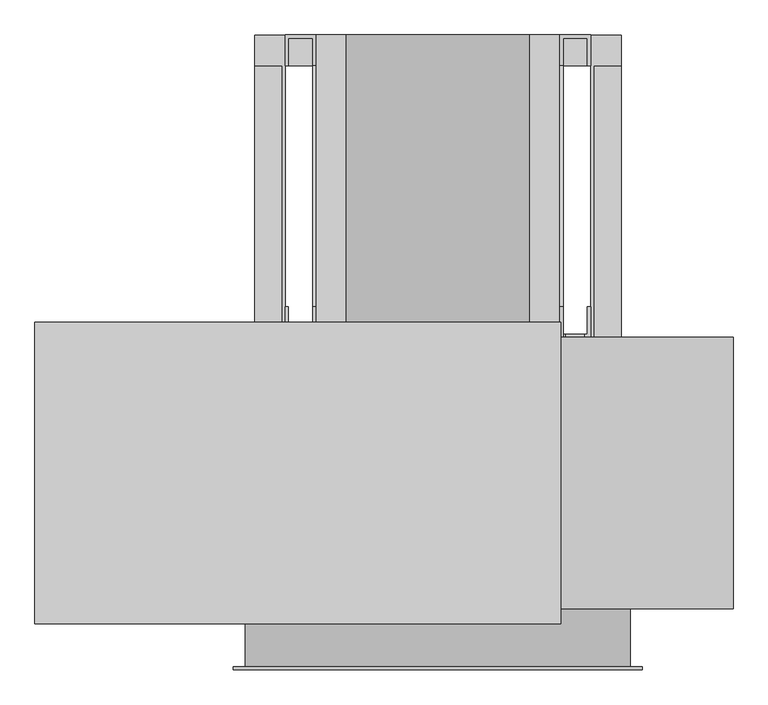
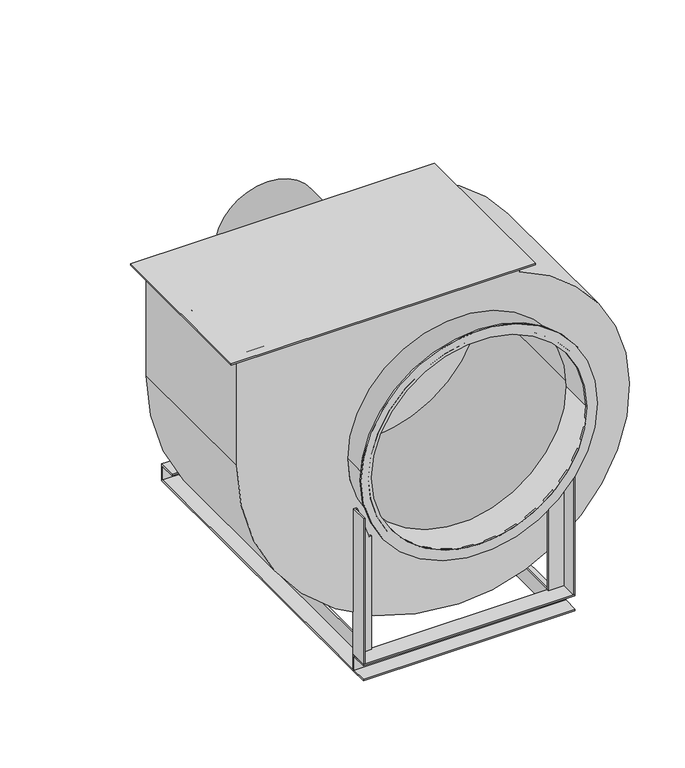
"""IFC4 building model written with IfcOpenShell, lengths in millimetres: proxy geometry, ВЕЗА_Вентилятор ВРАН : ВРАН6-063-ПО."""

from ifc_helpers import new_model, si_unit, point, frame, frame_2d, origin, place, context, project, spatial, polyline, circle_curve, trimmed, segment, composite_curve, outline, extrude, faceted_brep, source, transform, mapped, element, save


def mechanical_equipment_27ed4517(model_context):
    return source(origin(), model_context, "Body", "SolidModel", [
        extrude(outline(polyline([(201.5, 247.0), (201.5, -247.0), (-659.5, -247.0), (-659.5, 247.0), (201.5, 247.0)])), frame((0.0, 0.0, 1055.0), z_axis=(0.0, 0.0, 1.0), x_axis=(1.0, 0.0, 0.0)), (0.0, 0.0, 1.0), 5.0),
        extrude(outline(composite_curve([segment(trimmed(circle_curve(frame_2d((730.0, 5.524027)), 635.024027), [point((730.0, -629.5))], [point((95.0, 0.0))], False, "CARTESIAN"), True, "CONTINUOUS"), segment(trimmed(circle_curve(frame_2d((578.1699763, 0.3189338)), 483.1700816), [point((95.0, 0.0))], [point((1030.0, 171.5))], False, "CARTESIAN"), True, "CONTINUOUS"), segment(polyline([(1030.0, 171.5), (1060.0, 171.5), (1060.0, -629.5), (730.0, -629.5)]), True, "CONTINUOUS")], self_intersect=False), holes=[composite_curve([segment(trimmed(circle_curve(frame_2d((640.0, 0.0)), 315.0), [point((640.0, -315.0))], [point((640.0, 315.0))], True, "CARTESIAN"), True, "CONTINUOUS"), segment(trimmed(circle_curve(frame_2d((640.0, 0.0)), 315.0), [point((640.0, 315.0))], [point((640.0, -315.0))], True, "CARTESIAN"), True, "CONTINUOUS")], self_intersect=False)]), frame((0.0, -222.0, 0.0), z_axis=(0.0, 1.0, 0.0), x_axis=(0.0, 0.0, 1.0)), (0.0, 0.0, 1.0), 444.0),
        faceted_brep([(-300.0, 712.0, 5.0), (-300.0, 712.0, 45.0), (-300.0, 667.0, 45.0), (-300.0, 667.0, 50.0), (-300.0, 717.0, 50.0), (-300.0, 717.0, 0.0), (-300.0, -222.0, 0.0), (-300.0, -222.0, 5.0), (300.0, 717.0, 50.0), (300.0, 667.0, 50.0), (300.0, 667.0, 45.0), (300.0, 712.0, 45.0), (300.0, 712.0, 5.0), (300.0, -222.0, 5.0), (300.0, -222.0, 0.0), (300.0, 717.0, 0.0), (250.0, -222.0, 0.0), (250.0, 667.0, 0.0), (-250.0, 667.0, 0.0), (-250.0, -222.0, 0.0), (-255.0, 667.0, 45.0), (-255.0, 667.0, 50.0), (255.0, 667.0, 50.0), (255.0, 667.0, 45.0), (-200.0, 667.0, 490.0), (-205.0, 667.0, 490.0), (-205.0, 667.0, 50.0), (-245.0, 667.0, 50.0), (-245.0, 667.0, 490.0), (-250.0, 667.0, 490.0), (-250.0, 667.0, 50.0), (250.0, 667.0, 50.0), (250.0, 667.0, 490.0), (245.0, 667.0, 490.0), (245.0, 667.0, 50.0), (205.0, 667.0, 50.0), (205.0, 667.0, 490.0), (200.0, 667.0, 490.0), (200.0, 667.0, 50.0), (-200.0, 667.0, 50.0), (205.0, 667.0, 5.0), (205.0, 667.0, 45.0), (245.0, 667.0, 45.0), (245.0, 667.0, 5.0), (-245.0, 667.0, 5.0), (-245.0, 667.0, 45.0), (-205.0, 667.0, 45.0), (-205.0, 667.0, 5.0), (-200.0, 667.0, 5.0), (-200.0, 667.0, 45.0), (200.0, 667.0, 45.0), (200.0, 667.0, 5.0), (245.0, 712.0, 5.0), (205.0, 712.0, 5.0), (-205.0, 712.0, 5.0), (-245.0, 712.0, 5.0), (200.0, 712.0, 5.0), (-200.0, 712.0, 5.0), (255.0, -222.0, 5.0), (255.0, 712.0, 5.0), (-255.0, -222.0, 5.0), (-255.0, 712.0, 5.0), (-255.0, 712.0, 45.0), (255.0, 712.0, 45.0), (245.0, 712.0, 45.0), (205.0, 712.0, 45.0), (-205.0, 712.0, 45.0), (-245.0, 712.0, 45.0), (200.0, 712.0, 45.0), (-200.0, 712.0, 45.0), (-255.0, -222.0, 50.0), (-250.0, -222.0, 50.0), (-250.0, 717.0, 50.0), (250.0, 717.0, 50.0), (250.0, -222.0, 50.0), (255.0, -222.0, 50.0), (-205.0, 712.0, 50.0), (-245.0, 712.0, 50.0), (245.0, 712.0, 50.0), (205.0, 712.0, 50.0), (200.0, 717.0, 50.0), (-200.0, 717.0, 50.0), (-250.0, 717.0, 490.0), (-200.0, 717.0, 490.0), (200.0, 717.0, 490.0), (250.0, 717.0, 490.0), (-245.0, 712.0, 490.0), (-205.0, 712.0, 490.0), (205.0, 712.0, 490.0), (245.0, 712.0, 490.0)], [[[0, 1, 2, 3, 4, 5, 6, 7]], [[8, 9, 10, 11, 12, 13, 14, 15]], [[14, 16, 17, 18, 19, 6, 5, 15]], [[3, 2, 20, 21]], [[10, 9, 22, 23]], [[24, 25, 26, 27, 28, 29, 30, 18, 17, 31, 32, 33, 34, 35, 36, 37, 38, 39], [40, 41, 42, 43], [44, 45, 46, 47], [48, 49, 50, 51]], [[40, 43, 52, 53]], [[44, 47, 54, 55]], [[48, 51, 56, 57]], [[58, 13, 12, 59]], [[7, 60, 61, 0]], [[1, 0, 61, 62]], [[12, 11, 63, 59]], [[53, 52, 64, 65]], [[55, 54, 66, 67]], [[57, 56, 68, 69]], [[2, 1, 62, 20]], [[11, 10, 23, 63]], [[65, 64, 42, 41]], [[67, 66, 46, 45]], [[69, 68, 50, 49]], [[4, 3, 21, 70, 71, 30, 72]], [[9, 8, 73, 31, 74, 75, 22]], [[27, 26, 76, 77]], [[35, 34, 78, 79]], [[39, 38, 80, 81]], [[8, 15, 5, 4, 72, 82, 83, 81, 80, 84, 85, 73]], [[75, 74, 16, 14, 13, 58]], [[75, 58, 59, 63, 23, 22]], [[16, 74, 31, 17]], [[70, 60, 7, 6, 19, 71]], [[60, 70, 21, 20, 62, 61]], [[71, 19, 18, 30]], [[83, 82, 29, 28, 86, 87, 25, 24]], [[84, 37, 36, 88, 89, 33, 32, 85]], [[89, 88, 79, 78]], [[43, 42, 64, 52]], [[33, 89, 78, 34]], [[85, 32, 31, 73]], [[51, 50, 68, 56]], [[37, 84, 80, 38]], [[41, 40, 53, 65]], [[88, 36, 35, 79]], [[29, 82, 72, 30]], [[45, 44, 55, 67]], [[86, 28, 27, 77]], [[87, 86, 77, 76]], [[47, 46, 66, 54]], [[25, 87, 76, 26]], [[49, 48, 57, 69]], [[83, 24, 39, 81]]]),
        extrude(outline(polyline([(667.0, 0.0), (222.0, 0.0), (222.0, 840.0), (272.0420316, 840.0), (667.0, 530.0420316), (667.0, 0.0)]), holes=[polyline([(272.0, 515.0), (587.0, 515.0), (587.0, 521.5949723), (296.9504813, 740.0), (272.0, 740.0), (272.0, 515.0)])]), frame((-205.0, 0.0, 0.0), z_axis=(1.0, 0.0, 0.0), x_axis=(0.0, 1.0, 0.0)), (0.0, 0.0, 1.0), 5.0),
        faceted_brep([(250.0, -222.0, 50.0), (300.0, -222.0, 50.0), (300.0, -272.0, 50.0), (295.0, -272.0, 50.0), (295.0, -227.0, 50.0), (250.0, -227.0, 50.0), (250.0, -222.0, 390.0), (258.2904546, -222.0, 390.0), (289.966699, -222.0, 485.0), (300.0, -222.0, 485.0), (300.0, -272.0, 485.0), (295.0, -272.0, 485.0), (295.0, -227.0, 485.0), (289.966699, -227.0, 485.0), (258.2904546, -227.0, 390.0), (250.0, -227.0, 390.0)], [[[0, 1, 2, 3, 4, 5]], [[1, 0, 6, 7, 8, 9]], [[2, 1, 9, 10]], [[3, 2, 10, 11]], [[4, 3, 11, 12]], [[5, 4, 12, 13, 14, 15]], [[0, 5, 15, 6]], [[14, 7, 6, 15]], [[7, 14, 13, 8]], [[8, 13, 12, 11, 10, 9]]]),
        faceted_brep([(-250.0, -222.0, 50.0), (-250.0, -227.0, 50.0), (-295.0, -227.0, 50.0), (-295.0, -272.0, 50.0), (-300.0, -272.0, 50.0), (-300.0, -222.0, 50.0), (-250.0, -222.0, 390.0), (-250.0, -227.0, 390.0), (-258.2904546, -227.0, 390.0), (-289.966699, -227.0, 485.0), (-295.0, -227.0, 485.0), (-295.0, -272.0, 485.0), (-300.0, -272.0, 485.0), (-300.0, -222.0, 485.0), (-289.966699, -222.0, 485.0), (-258.2904546, -222.0, 390.0)], [[[0, 1, 2, 3, 4, 5]], [[1, 0, 6, 7]], [[2, 1, 7, 8, 9, 10]], [[3, 2, 10, 11]], [[4, 3, 11, 12]], [[5, 4, 12, 13]], [[0, 5, 13, 14, 15, 6]], [[9, 14, 13, 12, 11, 10]], [[14, 9, 8, 15]], [[15, 8, 7, 6]]]),
        extrude(outline(polyline([(667.0, 0.0), (222.0, 0.0), (222.0, 840.0), (272.0420316, 840.0), (667.0, 530.0420316), (667.0, 0.0)]), holes=[polyline([(272.0, 515.0), (587.0, 515.0), (587.0, 521.5949723), (296.9504813, 740.0), (272.0, 740.0), (272.0, 515.0)])]), frame((200.0, 0.0, 0.0), z_axis=(1.0, 0.0, 0.0), x_axis=(0.0, 1.0, 0.0)), (0.0, 0.0, 1.0), 5.0),
        faceted_brep([(200.0, 222.0, 0.0), (200.0, 227.0, 0.0), (245.0, 227.0, 0.0), (245.0, 272.0, 0.0), (250.0, 272.0, 0.0), (250.0, 222.0, 0.0), (250.0, 222.0, 750.0), (240.0, 222.0, 750.0), (208.75409, 222.0, 833.6095143), (200.0, 222.0, 833.6095143), (250.0, 272.0, 750.0), (245.0, 272.0, 750.0), (245.0, 227.0, 750.0), (200.0, 227.0, 833.6095143), (208.75409, 227.0, 833.6095143), (240.0, 227.0, 750.0)], [[[0, 1, 2, 3, 4, 5]], [[0, 5, 6, 7, 8, 9]], [[5, 4, 10, 6]], [[4, 3, 11, 10]], [[3, 2, 12, 11]], [[2, 1, 13, 14, 15, 12]], [[1, 0, 9, 13]], [[8, 14, 13, 9]], [[14, 8, 7, 15]], [[15, 7, 6, 10, 11, 12]]]),
        faceted_brep([(-200.0, 222.0, 0.0), (-250.0, 222.0, 0.0), (-250.0, 272.0, 0.0), (-245.0, 272.0, 0.0), (-245.0, 227.0, 0.0), (-200.0, 227.0, 0.0), (-200.0, 227.0, 833.6095143), (-200.0, 222.0, 833.6095143), (-245.0, 227.0, 750.0), (-240.0, 227.0, 750.0), (-208.75409, 227.0, 833.6095143), (-245.0, 272.0, 750.0), (-250.0, 272.0, 750.0), (-250.0, 222.0, 750.0), (-208.75409, 222.0, 833.6095143), (-240.0, 222.0, 750.0)], [[[0, 1, 2, 3, 4, 5]], [[0, 5, 6, 7]], [[5, 4, 8, 9, 10, 6]], [[4, 3, 11, 8]], [[3, 2, 12, 11]], [[2, 1, 13, 12]], [[1, 0, 7, 14, 15, 13]], [[15, 9, 8, 11, 12, 13]], [[9, 15, 14, 10]], [[10, 14, 7, 6]]]),
        extrude(outline(polyline([(-222.0, 50.0), (-222.0, 0.0), (-272.0, 0.0), (-272.0, 5.0), (-227.0, 5.0), (-227.0, 45.0), (-272.0, 45.0), (-272.0, 50.0), (-222.0, 50.0)])), frame((-300.0, 0.0, 0.0), z_axis=(1.0, 0.0, 0.0), x_axis=(0.0, 1.0, 0.0)), (0.0, 0.0, 1.0), 600.0),
        extrude(outline(composite_curve([segment(trimmed(circle_curve(frame_2d((640.0, 0.0)), 315.0), [point((640.0, -315.0))], [point((640.0, 315.0))], False, "CARTESIAN"), True, "CONTINUOUS"), segment(trimmed(circle_curve(frame_2d((640.0, 0.0)), 315.0), [point((640.0, 315.0))], [point((640.0, -315.0))], False, "CARTESIAN"), True, "CONTINUOUS")], self_intersect=False)), frame((0.0, 217.0, 0.0), z_axis=(0.0, 1.0, 0.0), x_axis=(0.0, 0.0, 1.0)), (0.0, 0.0, 1.0), 5.0),
        extrude(outline(composite_curve([segment(trimmed(circle_curve(frame_2d((640.0, 0.0)), 335.0), [point((640.0, -335.0))], [point((640.0, 335.0))], False, "CARTESIAN"), True, "CONTINUOUS"), segment(trimmed(circle_curve(frame_2d((640.0, 0.0)), 335.0), [point((640.0, 335.0))], [point((640.0, -335.0))], False, "CARTESIAN"), True, "CONTINUOUS")], self_intersect=False), holes=[composite_curve([segment(trimmed(circle_curve(frame_2d((640.0, 0.0)), 305.0), [point((640.0, -305.0))], [point((640.0, 305.0))], True, "CARTESIAN"), True, "CONTINUOUS"), segment(trimmed(circle_curve(frame_2d((640.0, 0.0)), 305.0), [point((640.0, 305.0))], [point((640.0, -305.0))], True, "CARTESIAN"), True, "CONTINUOUS")], self_intersect=False)]), frame((0.0, -322.0, 0.0), z_axis=(0.0, 1.0, 0.0), x_axis=(0.0, 0.0, 1.0)), (0.0, 0.0, 1.0), 5.0),
        extrude(outline(polyline([(200.0, 717.0), (200.0, 222.0), (-200.0, 222.0), (-200.0, 717.0), (200.0, 717.0)])), frame((0.0, 0.0, 440.0), z_axis=(0.0, 0.0, 1.0), x_axis=(1.0, 0.0, 0.0)), (0.0, 0.0, 1.0), 50.0),
        extrude(outline(composite_curve([segment(trimmed(circle_curve(frame_2d((640.0, 0.0)), 150.0), [point((640.0, 150.0))], [point((640.0, -150.0))], False, "CARTESIAN"), True, "CONTINUOUS"), segment(trimmed(circle_curve(frame_2d((640.0, 0.0)), 150.0), [point((640.0, -150.0))], [point((640.0, 150.0))], False, "CARTESIAN"), True, "CONTINUOUS")], self_intersect=False)), frame((0.0, 222.0, 0.0), z_axis=(0.0, 1.0, 0.0), x_axis=(0.0, 0.0, 1.0)), (0.0, 0.0, 1.0), 495.0),
        extrude(outline(composite_curve([segment(trimmed(circle_curve(frame_2d((640.0, 0.0)), 315.0), [point((640.0, 315.0))], [point((640.0, -315.0))], False, "CARTESIAN"), True, "CONTINUOUS"), segment(trimmed(circle_curve(frame_2d((640.0, 0.0)), 315.0), [point((640.0, -315.0))], [point((640.0, 315.0))], False, "CARTESIAN"), True, "CONTINUOUS")], self_intersect=False), holes=[composite_curve([segment(trimmed(circle_curve(frame_2d((640.0, 0.0)), 305.0), [point((640.0, 305.0))], [point((640.0, -305.0))], True, "CARTESIAN"), True, "CONTINUOUS"), segment(trimmed(circle_curve(frame_2d((640.0, 0.0)), 305.0), [point((640.0, -305.0))], [point((640.0, 305.0))], True, "CARTESIAN"), True, "CONTINUOUS")], self_intersect=False)]), frame((0.0, -322.0, 0.0), z_axis=(0.0, 1.0, 0.0), x_axis=(0.0, 0.0, 1.0)), (0.0, 0.0, 1.0), 100.0),
    ])


if __name__ == "__main__":
    model = new_model("IFC4")
    model_context = context("Model", 3, world=origin())
    ifc_project = project(units=[si_unit("LENGTHUNIT", "METRE", prefix="MILLI")], contexts=[model_context])
    site = spatial("IfcSite", under=ifc_project)
    building = spatial("IfcBuilding", under=site)
    placement = place(None, origin())
    mechanical_equipment_shape = mechanical_equipment_27ed4517(model_context)
    element("IfcBuildingElementProxy", 1, Name="ВЕЗА_Вентилятор ВРАН : ВРАН6-063-ПО", ObjectType="ВЕЗА_Вентилятор ВРАН : ВРАН6-063-ПО", at=placement, inside=building, context=model_context, shape_type="MappedRepresentation", body=[
        mapped(mechanical_equipment_shape, transform((0.0, 0.0, 0.0), x_axis=(1.0, 0.0, 0.0), y_axis=(0.0, 1.0, 0.0), z_axis=(0.0, 0.0, 1.0))),
    ])
    save(model, "model.ifc")

# Revit data of these elements
# Type "ВЕЗА_Вентилятор ВРАН : ВРАН6-063-ПО"
#   УголВысота = "ВРАН_Угол_Высота"
#   ADSK_Этаж [instance default] = ""
#   ADSK_Примечание [instance default] = ""
#   ADSK_Позиция = "11"
#   ADSK_Обозначение = ""
#   ADSK_Наименование = "Вентилятор радиальный ВРАН6; типоразмер 063; режим работы Т80; исполнение коррозионностойкое; номинальная мощность Nном=4кВт, число -2007 полюсов 4; климатическое исполнение \r\nУХЛ2; конструктивное исполнение 1; положение корпуса ПО; без ТШК"
#   О_Назначение [instance default] = ""
#   ADSK_Марка = "ВРАН6-063-Т80-К1 -00400/4-УХЛ2-1-ПО-О ТУ4861-104-40149153"
#   ADSK_Комплект [instance default] = ""
#   ADSK_Код изделия = "4044810"
#   ADSK_Зона [instance default] = ""
#   ADSK_Единица измерения = "компл."
#   И_НаименованиеФитинга = ""
#   И_НаименованиеСистемы [instance default] = ""
#   И_КодОборудования = "ВРАН6-063-ПД"
#   ADSK_Завод-изготовитель = "ООО \"Веза\", Россия, Москва, ИНН 505001001, info@veza.ru"
#   Габариты = "vran_du"
#   ШиринаСтойкиОкна2 = 100 mm
#   ШиринаСтойкиОкна1 = 130 mm
#   ШиринаСтойкиДвигателя = 50 mm
#   Уголок = 50 mm
#   УголНаклона [instance default] = 0°
#   Угол [instance default] = 0°
#   Столик = -50 mm
#   Расход [instance default] = 4000 m³/h
#   ADSK_Масса = 160
#   ADSK_Количество = 1
#   ADSK_Номинальная мощность [instance default] = 3000 W
#   РадиусДвигателя = 150 mm
#   НомерВентилятора = 6.3 mm
#   ВысотаПлощадкиДвигателя [instance default] = 490 mm
#   ВерхОпор = 200 mm
#   R3 = 335 mm
#   R2 = 305 mm
#   Lmax = 989 mm
#   h [instance default] = 640 mm
#   R = 315 mm
#   L2 = 231 mm
#   H = 1066 mm
#   D = 630 mm
#   C = 550 mm
#   B_корпуса = 1140 mm
#   B = 802 mm
#   A = 444 mm
#   Швеллер = yes
#   Default Elevation = 0
#   Type Comments = ""
